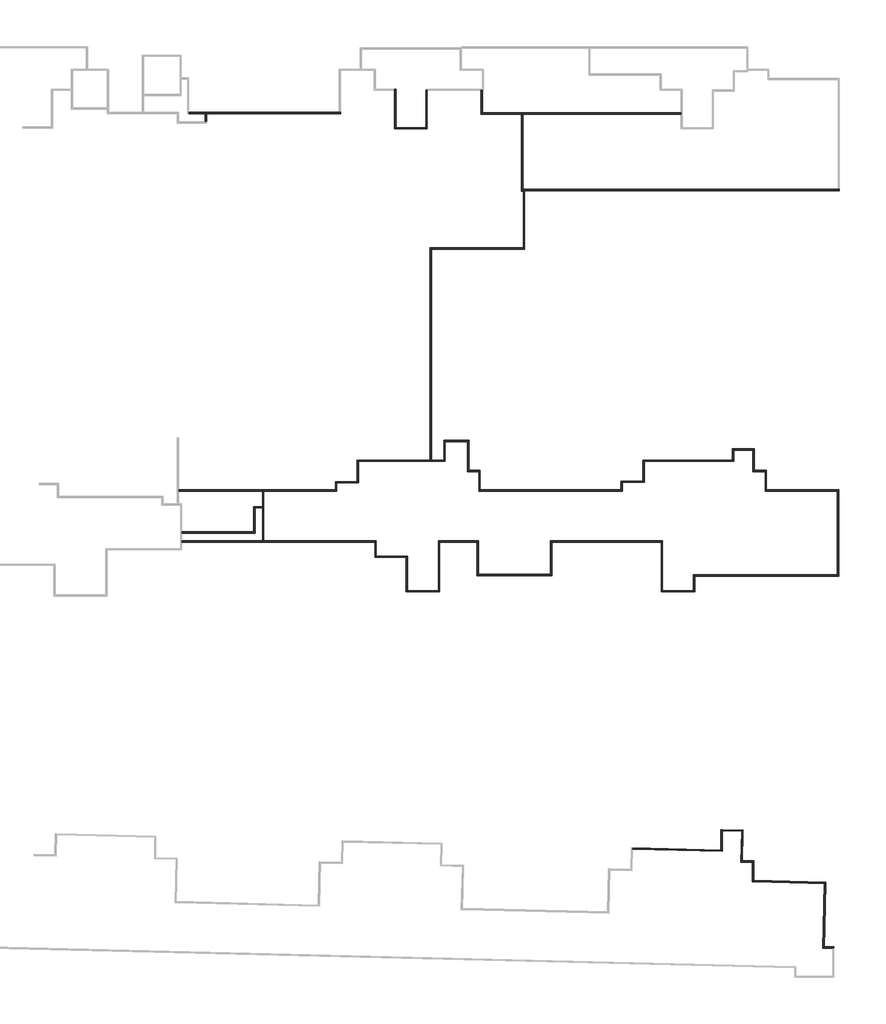
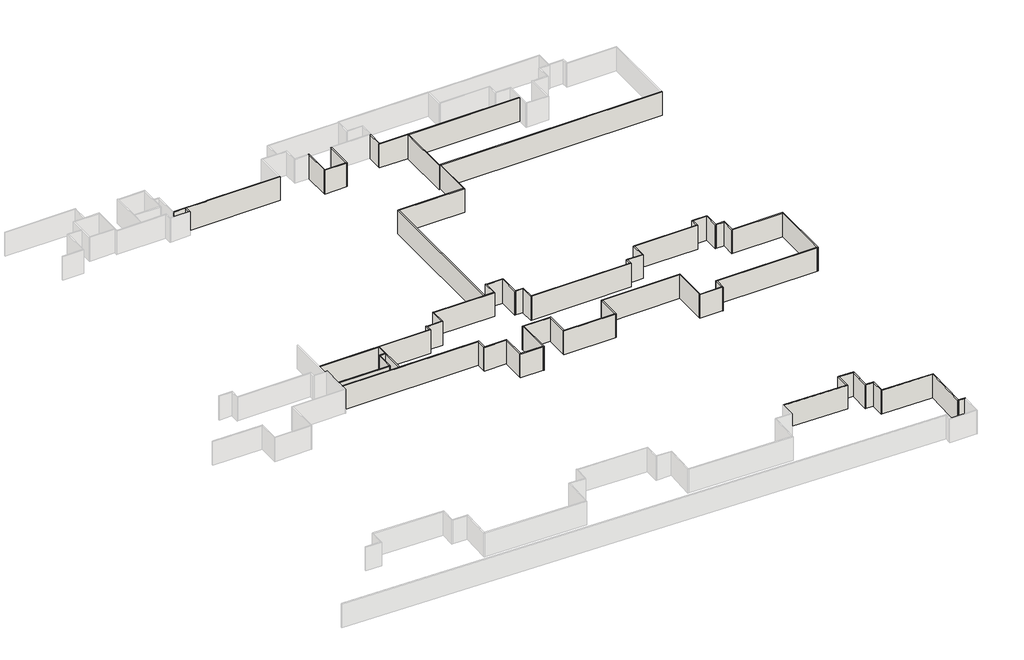
# One storey, part 7 of 8: 62 walls.
"""IFC4 building model written with IfcOpenShell, lengths in millimetres."""

from ifc_helpers import new_model, si_unit, origin, origin_with_axes, place, context, project, spatial, polyline, outline, extrude, faceted_brep, element, save

model = new_model("IFC4")

# Units and contexts
model_context = context("Model", 3, world=origin())
ifc_project = project(units=[si_unit("LENGTHUNIT", "METRE", prefix="MILLI")], contexts=[model_context])

# Site, building, storey
site = spatial("IfcSite", under=ifc_project)
building = spatial("IfcBuilding", under=site)
storey = spatial("IfcBuildingStorey", under=building, Name="户型图", Elevation=0.0)

# Walls
placement = place(None, origin())
element("IfcWall", 1, ObjectType="所有墙体", at=placement, inside=storey, context=model_context, shape_type="Brep", body=[
    faceted_brep([(295975.4891356, 26343.647248, 0.0), (304289.7878262, 26139.3963633, 0.0), (304289.7878262, 26139.3963633, 3300.0), (295975.4891356, 26343.647248, 3300.0), (295978.4361928, 26463.6110544, 0.0), (295978.4361928, 26463.6110544, 3300.0), (304169.7878262, 26262.3805141, 3300.0), (304289.7878262, 26259.4325678, 3300.0), (304289.7878262, 26259.4325678, 0.0), (304169.7878262, 26262.3805141, 0.0)], [[[0, 1, 2, 3]], [[4, 5, 6, 7, 8, 9]], [[1, 0, 4, 9, 8]], [[3, 2, 7, 6, 5]], [[0, 3, 5, 4]], [[2, 1, 8, 7]]]),
])
element("IfcWall", 2, ObjectType="所有墙体", at=placement, inside=storey, context=model_context, shape_type="Brep", body=[
    faceted_brep([(304289.7878262, 26259.4325678, 0.0), (304289.7878262, 28039.3963633, 0.0), (304289.7878262, 28159.4325678, 0.0), (304289.7878262, 28159.4325678, 3300.0), (304289.7878262, 28039.3963633, 3300.0), (304289.7878262, 26259.4325678, 3300.0), (304169.7878262, 26262.3805141, 0.0), (304169.7878262, 26262.3805141, 3300.0), (304169.7878262, 28162.3805141, 3300.0), (304169.7878262, 28162.3805141, 0.0)], [[[0, 1, 2, 3, 4, 5]], [[6, 7, 8, 9]], [[2, 1, 0, 6, 9]], [[5, 4, 3, 8, 7]], [[0, 5, 7, 6]], [[3, 2, 9, 8]]]),
])
element("IfcWall", 3, ObjectType="所有墙体", at=placement, inside=storey, context=model_context, shape_type="Brep", body=[
    faceted_brep([(304289.7878262, 28039.3963633, 0.0), (306114.4401038, 27994.5715553, 0.0), (306234.4039102, 27991.6244981, 0.0), (306234.4039102, 27991.6244981, 3300.0), (306114.4401038, 27994.5715553, 3300.0), (304289.7878262, 28039.3963633, 3300.0), (304289.7878262, 28159.4325678, 0.0), (304289.7878262, 28159.4325678, 3300.0), (306237.3509674, 28111.5883046, 3300.0), (306237.3509674, 28111.5883046, 0.0)], [[[0, 1, 2, 3, 4, 5]], [[6, 7, 8, 9]], [[2, 1, 0, 6, 9]], [[5, 4, 3, 8, 7]], [[0, 5, 7, 6]], [[3, 2, 9, 8]]]),
])
element("IfcWall", 4, ObjectType="所有墙体", at=placement, inside=storey, context=model_context, shape_type="Brep", body=[
    faceted_brep([(306114.4401038, 27994.5715553, 0.0), (306044.4174031, 25144.2061839, 0.0), (306044.4174031, 25144.2061839, 3300.0), (306114.4401038, 27994.5715553, 3300.0), (306234.4039102, 27991.6244981, 0.0), (306234.4039102, 27991.6244981, 3300.0), (306167.4015539, 25264.2061839, 3300.0), (306164.4536076, 25144.2061839, 3300.0), (306164.4536076, 25144.2061839, 0.0), (306167.4015539, 25264.2061839, 0.0)], [[[0, 1, 2, 3]], [[4, 5, 6, 7, 8, 9]], [[1, 0, 4, 9, 8]], [[3, 2, 7, 6, 5]], [[0, 3, 5, 4]], [[2, 1, 8, 7]]]),
])
element("IfcWall", 5, ObjectType="所有墙体", at=placement, inside=storey, context=model_context, shape_type="Brep", body=[
    faceted_brep([(306164.4536076, 25144.2061839, 0.0), (307105.9094785, 25144.2061839, 0.0), (307225.9094785, 25144.2061839, 0.0), (307225.9094785, 25144.2061839, 3300.0), (307105.9094785, 25144.2061839, 3300.0), (306164.4536076, 25144.2061839, 3300.0), (306167.4015539, 25264.2061839, 0.0), (306167.4015539, 25264.2061839, 3300.0), (307225.9094785, 25264.2061839, 3300.0), (307225.9094785, 25264.2061839, 0.0)], [[[0, 1, 2, 3, 4, 5]], [[6, 7, 8, 9]], [[2, 1, 0, 6, 9]], [[5, 4, 3, 8, 7]], [[0, 5, 7, 6]], [[3, 2, 9, 8]]]),
])
element("IfcWall", 6, ObjectType="所有墙体", at=placement, inside=storey, context=model_context, shape_type="Brep", body=[
    faceted_brep([(307105.9094785, 25144.2061839, 0.0), (307105.9094785, 23319.0782852, 0.0), (307105.9094785, 23319.0782852, 3300.0), (307105.9094785, 25144.2061839, 3300.0), (307225.9094785, 25144.2061839, 0.0), (307225.9094785, 25144.2061839, 3300.0), (307225.9094785, 23436.1665434, 3300.0), (307225.9094785, 23316.1303389, 3300.0), (307225.9094785, 23316.1303389, 0.0), (307225.9094785, 23436.1665434, 0.0)], [[[0, 1, 2, 3]], [[4, 5, 6, 7, 8, 9]], [[1, 0, 4, 9, 8]], [[3, 2, 7, 6, 5]], [[0, 3, 5, 4]], [[2, 1, 8, 7]]]),
])
element("IfcWall", 7, ObjectType="所有墙体", at=placement, inside=storey, context=model_context, shape_type="Brep", body=[
    faceted_brep([(307225.9094785, 23316.1303389, 0.0), (313802.4332392, 23154.5700142, 0.0), (313922.3970456, 23151.622957, 0.0), (313922.3970456, 23151.622957, 3300.0), (313802.4332392, 23154.5700142, 3300.0), (307225.9094785, 23316.1303389, 3300.0), (307225.9094785, 23436.1665434, 0.0), (307225.9094785, 23436.1665434, 3300.0), (313925.3441028, 23271.5867634, 3300.0), (313925.3441028, 23271.5867634, 0.0)], [[[0, 1, 2, 3, 4, 5]], [[6, 7, 8, 9]], [[2, 1, 0, 6, 9]], [[5, 4, 3, 8, 7]], [[0, 5, 7, 6]], [[3, 2, 9, 8]]]),
])
element("IfcWall", 8, ObjectType="所有墙体", at=placement, inside=storey, context=model_context, shape_type="Brep", body=[
    faceted_brep([(313802.4332392, 23154.5700142, 0.0), (313655.0436489, 17154.8844843, 0.0), (313655.0436489, 17154.8844843, 3300.0), (313802.4332392, 23154.5700142, 3300.0), (313922.3970456, 23151.622957, 0.0), (313922.3970456, 23151.622957, 3300.0), (313778.0277997, 17274.8844843, 3300.0), (313775.0798534, 17154.8844843, 3300.0), (313775.0798534, 17154.8844843, 0.0), (313778.0277997, 17274.8844843, 0.0)], [[[0, 1, 2, 3]], [[4, 5, 6, 7, 8, 9]], [[1, 0, 4, 9, 8]], [[3, 2, 7, 6, 5]], [[0, 3, 5, 4]], [[2, 1, 8, 7]]]),
])
element("IfcWall", 9, ObjectType="所有墙体", at=placement, inside=storey, context=model_context, shape_type="Brep", body=[
    faceted_brep([(313775.0798534, 17154.8844843, 0.0), (314556.5357243, 17154.8844843, 0.0), (314676.5357243, 17154.8844843, 0.0), (314676.5357243, 17154.8844843, 3300.0), (314556.5357243, 17154.8844843, 3300.0), (313775.0798534, 17154.8844843, 3300.0), (313778.0277997, 17274.8844843, 0.0), (313778.0277997, 17274.8844843, 3300.0), (314676.5357243, 17274.8844843, 3300.0), (314676.5357243, 17274.8844843, 0.0)], [[[0, 1, 2, 3, 4, 5]], [[6, 7, 8, 9]], [[2, 1, 0, 6, 9]], [[5, 4, 3, 8, 7]], [[0, 5, 7, 6]], [[3, 2, 9, 8]]]),
])
element("IfcWall", 10, ObjectType="所有墙体", at=placement, inside=storey, context=model_context, shape_type="SweptSolid", body=[
    extrude(outline(polyline([(256409.6849063, 94629.6848758), (256409.6849063, 93851.6486697), (256289.6849063, 93851.6486697), (256289.6849063, 94629.6848758), (256409.6849063, 94629.6848758)])), origin_with_axes(), (0.0, 0.0, 1.0), 3300.0),
])
element("IfcWall", 11, ObjectType="所有墙体", at=placement, inside=storey, context=model_context, shape_type="Brep", body=[
    faceted_brep([(254753.7757632, 94629.6848758, 0.0), (256289.6849063, 94629.6848758, 0.0), (256409.6849063, 94629.6848758, 0.0), (268831.7978195, 94629.6848758, 0.0), (268831.7978195, 94629.6848758, 2700.0), (268831.7978195, 94629.6848758, 3300.0), (268650.2438638, 94629.6848758, 3300.0), (259271.6890495, 94629.6848758, 3300.0), (258971.6890495, 94629.6848758, 3300.0), (256409.6849063, 94629.6848758, 3300.0), (256289.6849063, 94629.6848758, 3300.0), (254753.7757632, 94629.6848758, 3300.0), (254753.7757632, 94749.6848758, 0.0), (254753.7757632, 94749.6848758, 3300.0), (258971.6890495, 94749.6848758, 3300.0), (259271.6890495, 94749.6848758, 3300.0), (268711.7978195, 94749.6848758, 3300.0), (268831.7978195, 94749.6848758, 3300.0), (268831.7978195, 94749.6848758, 0.0), (268711.7978195, 94749.6848758, 0.0), (268831.7978195, 94694.4630172, 3300.0)], [[[0, 1, 2, 3, 4, 5, 6, 7, 8, 9, 10, 11]], [[12, 13, 14, 15, 16, 17, 18, 19]], [[3, 2, 1, 0, 12, 19, 18]], [[11, 10, 9, 8, 7, 6, 5, 20, 17, 16, 15, 14, 13]], [[5, 4, 3, 18, 17, 20]], [[0, 11, 13, 12]]]),
])
element("IfcWall", 12, ObjectType="所有墙体", at=placement, inside=storey, context=model_context, shape_type="Brep", body=[
    faceted_brep([(276761.765153, 96780.8975721, 0.0), (276761.765153, 93324.5302556, 0.0), (276761.765153, 93204.5302556, 0.0), (276761.765153, 93204.5302556, 3300.0), (276761.765153, 93324.5302556, 3300.0), (276761.765153, 96780.8975721, 3300.0), (276881.765153, 96780.8975721, 0.0), (276881.765153, 96780.8975721, 3300.0), (276881.765153, 93204.5302556, 3300.0), (276881.765153, 93204.5302556, 0.0)], [[[0, 1, 2, 3, 4, 5]], [[6, 7, 8, 9]], [[2, 1, 0, 6, 9]], [[5, 4, 3, 8, 7]], [[0, 5, 7, 6]], [[3, 2, 9, 8]]]),
])
element("IfcWall", 13, ObjectType="所有墙体", at=placement, inside=storey, context=model_context, shape_type="Brep", body=[
    faceted_brep([(276761.765153, 93324.5302556, 0.0), (273981.7651529, 93324.5302556, 0.0), (273861.7651529, 93324.5302556, 0.0), (273861.7651529, 93324.5302556, 3300.0), (273981.7651529, 93324.5302556, 3300.0), (276761.765153, 93324.5302556, 3300.0), (276761.765153, 93204.5302556, 0.0), (276761.765153, 93204.5302556, 3300.0), (273861.7651529, 93204.5302556, 3300.0), (273861.7651529, 93204.5302556, 0.0)], [[[0, 1, 2, 3, 4, 5]], [[6, 7, 8, 9]], [[2, 1, 0, 6, 9]], [[5, 4, 3, 8, 7]], [[0, 5, 7, 6]], [[3, 2, 9, 8]]]),
])
element("IfcWall", 14, ObjectType="所有墙体", at=placement, inside=storey, context=model_context, shape_type="Brep", body=[
    faceted_brep([(273981.7651529, 93324.5302556, 0.0), (273981.7651529, 96900.8975721, 0.0), (273981.7651529, 96900.8975721, 3300.0), (273981.7651529, 93324.5302556, 3300.0), (273861.7651529, 93324.5302556, 0.0), (273861.7651529, 93324.5302556, 3300.0), (273861.7651529, 96780.8975721, 3300.0), (273861.7651529, 96900.8975721, 3300.0), (273861.7651529, 96900.8975721, 0.0), (273861.7651529, 96780.8975721, 0.0)], [[[0, 1, 2, 3]], [[4, 5, 6, 7, 8, 9]], [[1, 0, 4, 9, 8]], [[3, 2, 7, 6, 5]], [[0, 3, 5, 4]], [[2, 1, 8, 7]]]),
])
element("IfcWall", 15, ObjectType="所有墙体", at=placement, inside=storey, context=model_context, shape_type="Brep", body=[
    faceted_brep([(253809.5875713, 59584.9975942, 0.0), (261588.0038327, 59584.9975942, 0.0), (261708.0038327, 59584.9975942, 0.0), (268485.4444886, 59584.9975942, 0.0), (268485.4444886, 59584.9975942, 3300.0), (261708.0038327, 59584.9975942, 3300.0), (261588.0038327, 59584.9975942, 3300.0), (253809.5875713, 59584.9975942, 3300.0), (253809.5875713, 59704.9975942, 0.0), (253809.5875713, 59704.9975942, 3300.0), (268365.4444886, 59704.9975942, 3300.0), (268485.4444886, 59704.9975942, 3300.0), (268485.4444886, 59704.9975942, 0.0), (268365.4444886, 59704.9975942, 0.0)], [[[0, 1, 2, 3, 4, 5, 6, 7]], [[8, 9, 10, 11, 12, 13]], [[3, 2, 1, 0, 8, 13, 12]], [[7, 6, 5, 4, 11, 10, 9]], [[4, 3, 12, 11]], [[0, 7, 9, 8]]]),
])
element("IfcWall", 16, ObjectType="所有墙体", at=placement, inside=storey, context=model_context, shape_type="Brep", body=[
    faceted_brep([(268485.4444886, 59704.9975942, 0.0), (268485.4444886, 60340.720191, 0.0), (268485.4444886, 60460.720191, 0.0), (268485.4444886, 60460.720191, 3300.0), (268485.4444886, 60340.720191, 3300.0), (268485.4444886, 59704.9975942, 3300.0), (268365.4444886, 59704.9975942, 0.0), (268365.4444886, 59704.9975942, 3300.0), (268365.4444886, 60460.720191, 3300.0), (268365.4444886, 60460.720191, 0.0)], [[[0, 1, 2, 3, 4, 5]], [[6, 7, 8, 9]], [[2, 1, 0, 6, 9]], [[5, 4, 3, 8, 7]], [[0, 5, 7, 6]], [[3, 2, 9, 8]]]),
])
element("IfcWall", 17, ObjectType="所有墙体", at=placement, inside=storey, context=model_context, shape_type="Brep", body=[
    faceted_brep([(268485.4444886, 60340.720191, 0.0), (270499.7227035, 60340.720191, 0.0), (270499.7227035, 60340.720191, 3300.0), (268485.4444886, 60340.720191, 3300.0), (268485.4444886, 60460.720191, 0.0), (268485.4444886, 60460.720191, 3300.0), (270379.7227035, 60460.720191, 3300.0), (270499.7227035, 60460.720191, 3300.0), (270499.7227035, 60460.720191, 0.0), (270379.7227035, 60460.720191, 0.0)], [[[0, 1, 2, 3]], [[4, 5, 6, 7, 8, 9]], [[1, 0, 4, 9, 8]], [[3, 2, 7, 6, 5]], [[0, 3, 5, 4]], [[2, 1, 8, 7]]]),
])
element("IfcWall", 18, ObjectType="所有墙体", at=placement, inside=storey, context=model_context, shape_type="Brep", body=[
    faceted_brep([(270499.7227035, 60460.720191, 0.0), (270499.7227035, 62334.5735496, 0.0), (270499.7227035, 62454.5735496, 0.0), (270499.7227035, 62454.5735496, 3300.0), (270499.7227035, 62334.5735496, 3300.0), (270499.7227035, 60460.720191, 3300.0), (270379.7227035, 60460.720191, 0.0), (270379.7227035, 60460.720191, 3300.0), (270379.7227035, 62423.9001534, 3300.0), (270379.7227035, 62454.5735496, 3300.0), (270379.7227035, 62454.5735496, 2700.0), (270379.7227035, 62454.5735496, 0.0), (270432.8505841, 62454.5735496, 3300.0)], [[[0, 1, 2, 3, 4, 5]], [[6, 7, 8, 9, 10, 11]], [[2, 1, 0, 6, 11]], [[5, 4, 3, 12, 9, 8, 7]], [[0, 5, 7, 6]], [[3, 2, 11, 10, 9, 12]]]),
])
element("IfcWall", 19, ObjectType="所有墙体", at=placement, inside=storey, context=model_context, shape_type="Brep", body=[
    faceted_brep([(270499.7227035, 62334.5735496, 0.0), (278560.2344713, 62334.5735496, 0.0), (278560.2344713, 62334.5735496, 3300.0), (270499.7227035, 62334.5735496, 3300.0), (270499.7227035, 62454.5735496, 0.0), (270499.7227035, 62454.5735496, 3300.0), (277178.9838503, 62454.5735496, 3300.0), (277298.9838503, 62454.5735496, 3300.0), (278440.2344713, 62454.5735496, 3300.0), (278560.2344713, 62454.5735496, 3300.0), (278560.2344713, 62454.5735496, 0.0), (278440.2344713, 62454.5735496, 0.0), (277298.9838503, 62454.5735496, 0.0), (277178.9838503, 62454.5735496, 0.0)], [[[0, 1, 2, 3]], [[4, 5, 6, 7, 8, 9, 10, 11, 12, 13]], [[1, 0, 4, 13, 12, 11, 10]], [[3, 2, 9, 8, 7, 6, 5]], [[0, 3, 5, 4]], [[2, 1, 10, 9]]]),
])
element("IfcWall", 20, ObjectType="所有墙体", at=placement, inside=storey, context=model_context, shape_type="Brep", body=[
    faceted_brep([(278560.2344713, 62454.5735496, 0.0), (278560.2344713, 64182.3314748, 0.0), (278560.2344713, 64302.3314748, 0.0), (278560.2344713, 64302.3314748, 3300.0), (278560.2344713, 64182.3314748, 3300.0), (278560.2344713, 62454.5735496, 3300.0), (278440.2344713, 62454.5735496, 0.0), (278440.2344713, 62454.5735496, 3300.0), (278440.2344713, 64302.3314748, 3300.0), (278440.2344713, 64302.3314748, 0.0)], [[[0, 1, 2, 3, 4, 5]], [[6, 7, 8, 9]], [[2, 1, 0, 6, 9]], [[5, 4, 3, 8, 7]], [[0, 5, 7, 6]], [[3, 2, 9, 8]]]),
])
element("IfcWall", 21, ObjectType="所有墙体", at=placement, inside=storey, context=model_context, shape_type="Brep", body=[
    faceted_brep([(278560.2344713, 64182.3314748, 0.0), (280640.2541721, 64182.3314748, 0.0), (280760.2541721, 64182.3314748, 0.0), (280760.2541721, 64182.3314748, 3300.0), (280640.2541721, 64182.3314748, 3300.0), (278560.2344713, 64182.3314748, 3300.0), (278560.2344713, 64302.3314748, 0.0), (278560.2344713, 64302.3314748, 3300.0), (280760.2541721, 64302.3314748, 3300.0), (280760.2541721, 64302.3314748, 0.0)], [[[0, 1, 2, 3, 4, 5]], [[6, 7, 8, 9]], [[2, 1, 0, 6, 9]], [[5, 4, 3, 8, 7]], [[0, 5, 7, 6]], [[3, 2, 9, 8]]]),
])
element("IfcWall", 22, ObjectType="所有墙体", at=placement, inside=storey, context=model_context, shape_type="Brep", body=[
    faceted_brep([(280640.2541721, 64182.3314748, 0.0), (280640.2541721, 61382.33135, 0.0), (280640.2541721, 61382.33135, 3300.0), (280640.2541721, 64182.3314748, 3300.0), (280760.2541721, 64182.3314748, 0.0), (280760.2541721, 64182.3314748, 3300.0), (280760.2541721, 61502.33135, 3300.0), (280760.2541721, 61382.33135, 3300.0), (280760.2541721, 61382.33135, 0.0), (280760.2541721, 61502.33135, 0.0)], [[[0, 1, 2, 3]], [[4, 5, 6, 7, 8, 9]], [[1, 0, 4, 9, 8]], [[3, 2, 7, 6, 5]], [[0, 3, 5, 4]], [[2, 1, 8, 7]]]),
])
element("IfcWall", 23, ObjectType="所有墙体", at=placement, inside=storey, context=model_context, shape_type="Brep", body=[
    faceted_brep([(280760.2541721, 61382.33135, 0.0), (281690.234471, 61382.33135, 0.0), (281810.234471, 61382.33135, 0.0), (281810.234471, 61382.33135, 3300.0), (281690.234471, 61382.33135, 3300.0), (280760.2541721, 61382.33135, 3300.0), (280760.2541721, 61502.33135, 0.0), (280760.2541721, 61502.33135, 3300.0), (281810.234471, 61502.33135, 3300.0), (281810.234471, 61502.33135, 0.0)], [[[0, 1, 2, 3, 4, 5]], [[6, 7, 8, 9]], [[2, 1, 0, 6, 9]], [[5, 4, 3, 8, 7]], [[0, 5, 7, 6]], [[3, 2, 9, 8]]]),
])
element("IfcWall", 24, ObjectType="所有墙体", at=placement, inside=storey, context=model_context, shape_type="Brep", body=[
    faceted_brep([(281690.234471, 61382.33135, 0.0), (281690.234471, 59584.9975942, 0.0), (281690.234471, 59584.9975942, 3300.0), (281690.234471, 61382.33135, 3300.0), (281810.234471, 61382.33135, 0.0), (281810.234471, 61382.33135, 3300.0), (281810.234471, 59704.9975942, 3300.0), (281810.234471, 59584.9975942, 3300.0), (281810.234471, 59584.9975942, 0.0), (281810.234471, 59704.9975942, 0.0)], [[[0, 1, 2, 3]], [[4, 5, 6, 7, 8, 9]], [[1, 0, 4, 9, 8]], [[3, 2, 7, 6, 5]], [[0, 3, 5, 4]], [[2, 1, 8, 7]]]),
])
element("IfcWall", 25, ObjectType="所有墙体", at=placement, inside=storey, context=model_context, shape_type="Brep", body=[
    faceted_brep([(281810.234471, 59584.9975942, 0.0), (295010.2344624, 59584.9975942, 0.0), (295010.2344624, 59584.9975942, 3300.0), (281810.234471, 59584.9975942, 3300.0), (281810.234471, 59704.9975942, 0.0), (281810.234471, 59704.9975942, 3300.0), (294890.2344624, 59704.9975942, 3300.0), (295010.2344624, 59704.9975942, 3300.0), (295010.2344624, 59704.9975942, 0.0), (294890.2344624, 59704.9975942, 0.0)], [[[0, 1, 2, 3]], [[4, 5, 6, 7, 8, 9]], [[1, 0, 4, 9, 8]], [[3, 2, 7, 6, 5]], [[0, 3, 5, 4]], [[2, 1, 8, 7]]]),
])
element("IfcWall", 26, ObjectType="所有墙体", at=placement, inside=storey, context=model_context, shape_type="Brep", body=[
    faceted_brep([(295010.2344624, 59704.9975942, 0.0), (295010.2344624, 60382.7613824, 0.0), (295010.2344624, 60502.7613824, 0.0), (295010.2344624, 60502.7613824, 3300.0), (295010.2344624, 60382.7613824, 3300.0), (295010.2344624, 59704.9975942, 3300.0), (294890.2344624, 59704.9975942, 0.0), (294890.2344624, 59704.9975942, 3300.0), (294890.2344624, 60502.7613824, 3300.0), (294890.2344624, 60502.7613824, 0.0)], [[[0, 1, 2, 3, 4, 5]], [[6, 7, 8, 9]], [[2, 1, 0, 6, 9]], [[5, 4, 3, 8, 7]], [[0, 5, 7, 6]], [[3, 2, 9, 8]]]),
])
element("IfcWall", 27, ObjectType="所有墙体", at=placement, inside=storey, context=model_context, shape_type="Brep", body=[
    faceted_brep([(295010.2344624, 60382.7613824, 0.0), (297060.2344614, 60382.7613824, 0.0), (297060.2344614, 60382.7613824, 3300.0), (295010.2344624, 60382.7613824, 3300.0), (295010.2344624, 60502.7613824, 0.0), (295010.2344624, 60502.7613824, 3300.0), (296940.2344614, 60502.7613824, 3300.0), (297060.2344614, 60502.7613824, 3300.0), (297060.2344614, 60502.7613824, 0.0), (296940.2344614, 60502.7613824, 0.0)], [[[0, 1, 2, 3]], [[4, 5, 6, 7, 8, 9]], [[1, 0, 4, 9, 8]], [[3, 2, 7, 6, 5]], [[0, 3, 5, 4]], [[2, 1, 8, 7]]]),
])
element("IfcWall", 28, ObjectType="所有墙体", at=placement, inside=storey, context=model_context, shape_type="Brep", body=[
    faceted_brep([(297060.2344614, 60502.7613824, 0.0), (297060.2344614, 62334.5735496, 0.0), (297060.2344614, 62454.5735496, 0.0), (297060.2344614, 62454.5735496, 3300.0), (297060.2344614, 62334.5735496, 3300.0), (297060.2344614, 60502.7613824, 3300.0), (296940.2344614, 60502.7613824, 0.0), (296940.2344614, 60502.7613824, 3300.0), (296940.2344614, 62454.5735496, 3300.0), (296940.2344614, 62454.5735496, 0.0)], [[[0, 1, 2, 3, 4, 5]], [[6, 7, 8, 9]], [[2, 1, 0, 6, 9]], [[5, 4, 3, 8, 7]], [[0, 5, 7, 6]], [[3, 2, 9, 8]]]),
])
element("IfcWall", 29, ObjectType="所有墙体", at=placement, inside=storey, context=model_context, shape_type="Brep", body=[
    faceted_brep([(297060.2344614, 62334.5735496, 0.0), (305360.2304568, 62334.5735496, 0.0), (305360.2304568, 62334.5735496, 3300.0), (297060.2344614, 62334.5735496, 3300.0), (297060.2344614, 62454.5735496, 0.0), (297060.2344614, 62454.5735496, 3300.0), (305240.2304568, 62454.5735496, 3300.0), (305360.2304568, 62454.5735496, 3300.0), (305360.2304568, 62454.5735496, 0.0), (305240.2304568, 62454.5735496, 0.0)], [[[0, 1, 2, 3]], [[4, 5, 6, 7, 8, 9]], [[1, 0, 4, 9, 8]], [[3, 2, 7, 6, 5]], [[0, 3, 5, 4]], [[2, 1, 8, 7]]]),
])
element("IfcWall", 30, ObjectType="所有墙体", at=placement, inside=storey, context=model_context, shape_type="Brep", body=[
    faceted_brep([(305360.2304568, 62454.5735496, 0.0), (305360.2304568, 63382.3074511, 0.0), (305360.2304568, 63502.3074511, 0.0), (305360.2304568, 63502.3074511, 3300.0), (305360.2304568, 63382.3074511, 3300.0), (305360.2304568, 62454.5735496, 3300.0), (305240.2304568, 62454.5735496, 0.0), (305240.2304568, 62454.5735496, 3300.0), (305240.2304568, 63502.3074511, 3300.0), (305240.2304568, 63502.3074511, 0.0)], [[[0, 1, 2, 3, 4, 5]], [[6, 7, 8, 9]], [[2, 1, 0, 6, 9]], [[5, 4, 3, 8, 7]], [[0, 5, 7, 6]], [[3, 2, 9, 8]]]),
])
element("IfcWall", 31, ObjectType="所有墙体", at=placement, inside=storey, context=model_context, shape_type="Brep", body=[
    faceted_brep([(305360.2304568, 63382.3074511, 0.0), (307140.2304762, 63382.3074511, 0.0), (307260.2304762, 63382.3074511, 0.0), (307260.2304762, 63382.3074511, 3300.0), (307140.2304762, 63382.3074511, 3300.0), (305360.2304568, 63382.3074511, 3300.0), (305360.2304568, 63502.3074511, 0.0), (305360.2304568, 63502.3074511, 3300.0), (307260.2304762, 63502.3074511, 3300.0), (307260.2304762, 63502.3074511, 0.0)], [[[0, 1, 2, 3, 4, 5]], [[6, 7, 8, 9]], [[2, 1, 0, 6, 9]], [[5, 4, 3, 8, 7]], [[0, 5, 7, 6]], [[3, 2, 9, 8]]]),
])
element("IfcWall", 32, ObjectType="所有墙体", at=placement, inside=storey, context=model_context, shape_type="Brep", body=[
    faceted_brep([(307140.2304762, 63382.3074511, 0.0), (307140.2304762, 61382.3313458, 0.0), (307140.2304762, 61382.3313458, 3300.0), (307140.2304762, 63382.3074511, 3300.0), (307260.2304762, 63382.3074511, 0.0), (307260.2304762, 63382.3074511, 3300.0), (307260.2304762, 61502.3313458, 3300.0), (307260.2304762, 61382.3313458, 3300.0), (307260.2304762, 61382.3313458, 0.0), (307260.2304762, 61502.3313458, 0.0)], [[[0, 1, 2, 3]], [[4, 5, 6, 7, 8, 9]], [[1, 0, 4, 9, 8]], [[3, 2, 7, 6, 5]], [[0, 3, 5, 4]], [[2, 1, 8, 7]]]),
])
element("IfcWall", 33, ObjectType="所有墙体", at=placement, inside=storey, context=model_context, shape_type="Brep", body=[
    faceted_brep([(307260.2304762, 61382.3313458, 0.0), (308290.2344624, 61382.3313458, 0.0), (308410.2344624, 61382.3313458, 0.0), (308410.2344624, 61382.3313458, 3300.0), (308290.2344624, 61382.3313458, 3300.0), (307260.2304762, 61382.3313458, 3300.0), (307260.2304762, 61502.3313458, 0.0), (307260.2304762, 61502.3313458, 3300.0), (308410.2344624, 61502.3313458, 3300.0), (308410.2344624, 61502.3313458, 0.0)], [[[0, 1, 2, 3, 4, 5]], [[6, 7, 8, 9]], [[2, 1, 0, 6, 9]], [[5, 4, 3, 8, 7]], [[0, 5, 7, 6]], [[3, 2, 9, 8]]]),
])
element("IfcWall", 34, ObjectType="所有墙体", at=placement, inside=storey, context=model_context, shape_type="Brep", body=[
    faceted_brep([(308290.2344624, 61382.3313458, 0.0), (308290.2344624, 59584.9975942, 0.0), (308290.2344624, 59584.9975942, 3300.0), (308290.2344624, 61382.3313458, 3300.0), (308410.2344624, 61382.3313458, 0.0), (308410.2344624, 61382.3313458, 3300.0), (308410.2344624, 59704.9975942, 3300.0), (308410.2344624, 59584.9975942, 3300.0), (308410.2344624, 59584.9975942, 0.0), (308410.2344624, 59704.9975942, 0.0)], [[[0, 1, 2, 3]], [[4, 5, 6, 7, 8, 9]], [[1, 0, 4, 9, 8]], [[3, 2, 7, 6, 5]], [[0, 3, 5, 4]], [[2, 1, 8, 7]]]),
])
element("IfcWall", 35, ObjectType="所有墙体", at=placement, inside=storey, context=model_context, shape_type="Brep", body=[
    faceted_brep([(308410.2344624, 59584.9975942, 0.0), (314990.2344624, 59584.9975942, 0.0), (315110.2344624, 59584.9975942, 0.0), (315110.2344624, 59584.9975942, 3300.0), (314990.2344624, 59584.9975942, 3300.0), (308410.2344624, 59584.9975942, 3300.0), (308410.2344624, 59704.9975942, 0.0), (308410.2344624, 59704.9975942, 3300.0), (315110.2344624, 59704.9975942, 3300.0), (315110.2344624, 59704.9975942, 0.0)], [[[0, 1, 2, 3, 4, 5]], [[6, 7, 8, 9]], [[2, 1, 0, 6, 9]], [[5, 4, 3, 8, 7]], [[0, 5, 7, 6]], [[3, 2, 9, 8]]]),
])
element("IfcWall", 36, ObjectType="所有墙体", at=placement, inside=storey, context=model_context, shape_type="Brep", body=[
    faceted_brep([(314990.2344624, 59584.9975942, 0.0), (314990.2344624, 51802.3314613, 0.0), (314990.2344624, 51682.3314613, 0.0), (314990.2344624, 51682.3314613, 3300.0), (314990.2344624, 51802.3314613, 3300.0), (314990.2344624, 59584.9975942, 3300.0), (315110.2344624, 59584.9975942, 0.0), (315110.2344624, 59584.9975942, 3300.0), (315110.2344624, 51682.3314613, 3300.0), (315110.2344624, 51682.3314613, 0.0)], [[[0, 1, 2, 3, 4, 5]], [[6, 7, 8, 9]], [[2, 1, 0, 6, 9]], [[5, 4, 3, 8, 7]], [[0, 5, 7, 6]], [[3, 2, 9, 8]]]),
])
element("IfcWall", 37, ObjectType="所有墙体", at=placement, inside=storey, context=model_context, shape_type="Brep", body=[
    faceted_brep([(314990.2344624, 51802.3314613, 0.0), (301640.3717048, 51802.3314613, 0.0), (301640.3717048, 51802.3314613, 3300.0), (314990.2344624, 51802.3314613, 3300.0), (314990.2344624, 51682.3314613, 0.0), (314990.2344624, 51682.3314613, 3300.0), (301760.3717048, 51682.3314613, 3300.0), (301640.3717048, 51682.3314613, 3300.0), (301640.3717048, 51682.3314613, 0.0), (301760.3717048, 51682.3314613, 0.0)], [[[0, 1, 2, 3]], [[4, 5, 6, 7, 8, 9]], [[1, 0, 4, 9, 8]], [[3, 2, 7, 6, 5]], [[0, 3, 5, 4]], [[2, 1, 8, 7]]]),
])
element("IfcWall", 38, ObjectType="所有墙体", at=placement, inside=storey, context=model_context, shape_type="Brep", body=[
    faceted_brep([(301640.3717048, 51682.3314613, 0.0), (301640.3717048, 50352.3314615, 0.0), (301640.3717048, 50232.3314615, 0.0), (301640.3717048, 50232.3314615, 3300.0), (301640.3717048, 50352.3314615, 3300.0), (301640.3717048, 51682.3314613, 3300.0), (301760.3717048, 51682.3314613, 0.0), (301760.3717048, 51682.3314613, 3300.0), (301760.3717048, 50232.3314615, 3300.0), (301760.3717048, 50232.3314615, 0.0)], [[[0, 1, 2, 3, 4, 5]], [[6, 7, 8, 9]], [[2, 1, 0, 6, 9]], [[5, 4, 3, 8, 7]], [[0, 5, 7, 6]], [[3, 2, 9, 8]]]),
])
element("IfcWall", 39, ObjectType="所有墙体", at=placement, inside=storey, context=model_context, shape_type="Brep", body=[
    faceted_brep([(301640.3717048, 50352.3314615, 0.0), (298760.3716961, 50352.3314615, 0.0), (298640.3716961, 50352.3314615, 0.0), (298640.3716961, 50352.3314615, 3300.0), (298760.3716961, 50352.3314615, 3300.0), (301640.3717048, 50352.3314615, 3300.0), (301640.3717048, 50232.3314615, 0.0), (301640.3717048, 50232.3314615, 3300.0), (298640.3716961, 50232.3314615, 3300.0), (298640.3716961, 50232.3314615, 0.0)], [[[0, 1, 2, 3, 4, 5]], [[6, 7, 8, 9]], [[2, 1, 0, 6, 9]], [[5, 4, 3, 8, 7]], [[0, 5, 7, 6]], [[3, 2, 9, 8]]]),
])
element("IfcWall", 40, ObjectType="所有墙体", at=placement, inside=storey, context=model_context, shape_type="Brep", body=[
    faceted_brep([(298760.3716961, 50352.3314615, 0.0), (298760.3716961, 54952.3246977, 0.0), (298760.3716961, 54952.3246977, 3300.0), (298760.3716961, 50352.3314615, 3300.0), (298640.3716961, 50352.3314615, 0.0), (298640.3716961, 50352.3314615, 3300.0), (298640.3716961, 54832.3246977, 3300.0), (298640.3716961, 54952.3246977, 3300.0), (298640.3716961, 54952.3246977, 0.0), (298640.3716961, 54832.3246977, 0.0)], [[[0, 1, 2, 3]], [[4, 5, 6, 7, 8, 9]], [[1, 0, 4, 9, 8]], [[3, 2, 7, 6, 5]], [[0, 3, 5, 4]], [[2, 1, 8, 7]]]),
])
element("IfcWall", 41, ObjectType="所有墙体", at=placement, inside=storey, context=model_context, shape_type="Brep", body=[
    faceted_brep([(298640.3716961, 54952.3246977, 0.0), (288340.2344711, 54952.3246977, 0.0), (288340.2344711, 54952.3246977, 3300.0), (298640.3716961, 54952.3246977, 3300.0), (298640.3716961, 54832.3246977, 0.0), (298640.3716961, 54832.3246977, 3300.0), (288460.2344711, 54832.3246977, 3300.0), (288340.2344711, 54832.3246977, 3300.0), (288340.2344711, 54832.3246977, 0.0), (288460.2344711, 54832.3246977, 0.0)], [[[0, 1, 2, 3]], [[4, 5, 6, 7, 8, 9]], [[1, 0, 4, 9, 8]], [[3, 2, 7, 6, 5]], [[0, 3, 5, 4]], [[2, 1, 8, 7]]]),
])
element("IfcWall", 42, ObjectType="所有墙体", at=placement, inside=storey, context=model_context, shape_type="Brep", body=[
    faceted_brep([(288340.2344711, 54832.3246977, 0.0), (288340.2344711, 51852.3246977, 0.0), (288340.2344711, 51732.3246977, 0.0), (288340.2344711, 51732.3246977, 3300.0), (288340.2344711, 51852.3246977, 3300.0), (288340.2344711, 54832.3246977, 3300.0), (288460.2344711, 54832.3246977, 0.0), (288460.2344711, 54832.3246977, 3300.0), (288460.2344711, 51852.3246977, 3300.0), (288460.2344711, 51732.3246977, 3300.0), (288460.2344711, 51732.3246977, 2700.0), (288460.2344711, 51732.3246977, 0.0)], [[[0, 1, 2, 3, 4, 5]], [[6, 7, 8, 9, 10, 11]], [[2, 1, 0, 6, 11]], [[5, 4, 3, 9, 8, 7]], [[0, 5, 7, 6]], [[3, 2, 11, 10, 9]]]),
])
element("IfcWall", 43, ObjectType="所有墙体", at=placement, inside=storey, context=model_context, shape_type="Brep", body=[
    faceted_brep([(288340.2344711, 51852.3246977, 0.0), (281660.2344711, 51852.3246977, 0.0), (281540.2344711, 51852.3246977, 0.0), (281540.2344711, 51852.3246977, 3300.0), (281660.2344711, 51852.3246977, 3300.0), (288340.2344711, 51852.3246977, 3300.0), (288340.2344711, 51732.3246977, 0.0), (288340.2344711, 51732.3246977, 3300.0), (281663.9582145, 51732.3246977, 3300.0), (281540.2344711, 51732.3246977, 3300.0), (281540.2344711, 51732.3246977, 2700.0), (281540.2344711, 51732.3246977, 0.0), (281540.2344711, 51842.0227808, 3300.0)], [[[0, 1, 2, 3, 4, 5]], [[6, 7, 8, 9, 10, 11]], [[2, 1, 0, 6, 11]], [[5, 4, 3, 12, 9, 8, 7]], [[0, 5, 7, 6]], [[3, 2, 11, 10, 9, 12]]]),
])
element("IfcWall", 44, ObjectType="所有墙体", at=placement, inside=storey, context=model_context, shape_type="Brep", body=[
    faceted_brep([(281660.2344711, 51852.3246977, 0.0), (281660.2344711, 54952.3246977, 0.0), (281660.2344711, 54952.3246977, 3300.0), (281660.2344711, 51852.3246977, 3300.0), (281540.2344711, 51852.3246977, 0.0), (281540.2344711, 51852.3246977, 3300.0), (281540.2344711, 54832.3246977, 3300.0), (281540.2344711, 54952.3246977, 3300.0), (281540.2344711, 54952.3246977, 0.0), (281540.2344711, 54832.3246977, 0.0)], [[[0, 1, 2, 3]], [[4, 5, 6, 7, 8, 9]], [[1, 0, 4, 9, 8]], [[3, 2, 7, 6, 5]], [[0, 3, 5, 4]], [[2, 1, 8, 7]]]),
])
element("IfcWall", 45, ObjectType="所有墙体", at=placement, inside=storey, context=model_context, shape_type="Brep", body=[
    faceted_brep([(281540.2344711, 54952.3246977, 0.0), (277940.3720183, 54952.3246977, 0.0), (277940.3720183, 54952.3246977, 3300.0), (281540.2344711, 54952.3246977, 3300.0), (281540.2344711, 54832.3246977, 0.0), (281540.2344711, 54832.3246977, 3300.0), (278060.3720183, 54832.3246977, 3300.0), (277940.3720183, 54832.3246977, 3300.0), (277940.3720183, 54832.3246977, 0.0), (278060.3720183, 54832.3246977, 0.0)], [[[0, 1, 2, 3]], [[4, 5, 6, 7, 8, 9]], [[1, 0, 4, 9, 8]], [[3, 2, 7, 6, 5]], [[0, 3, 5, 4]], [[2, 1, 8, 7]]]),
])
element("IfcWall", 46, ObjectType="所有墙体", at=placement, inside=storey, context=model_context, shape_type="Brep", body=[
    faceted_brep([(277940.3720183, 54832.3246977, 0.0), (277940.3720183, 50352.3314615, 0.0), (277940.3720183, 50232.3314615, 0.0), (277940.3720183, 50232.3314615, 3300.0), (277940.3720183, 50352.3314615, 3300.0), (277940.3720183, 54832.3246977, 3300.0), (278060.3720183, 54832.3246977, 0.0), (278060.3720183, 54832.3246977, 3300.0), (278060.3720183, 50232.3314615, 3300.0), (278060.3720183, 50232.3314615, 0.0)], [[[0, 1, 2, 3, 4, 5]], [[6, 7, 8, 9]], [[2, 1, 0, 6, 9]], [[5, 4, 3, 8, 7]], [[0, 5, 7, 6]], [[3, 2, 9, 8]]]),
])
element("IfcWall", 47, ObjectType="所有墙体", at=placement, inside=storey, context=model_context, shape_type="Brep", body=[
    faceted_brep([(277940.3720183, 50352.3314615, 0.0), (275060.3720183, 50352.3314615, 0.0), (274940.3720183, 50352.3314615, 0.0), (274940.3720183, 50352.3314615, 3300.0), (275060.3720183, 50352.3314615, 3300.0), (277940.3720183, 50352.3314615, 3300.0), (277940.3720183, 50232.3314615, 0.0), (277940.3720183, 50232.3314615, 3300.0), (275149.8189959, 50232.3314615, 3300.0), (274940.3720183, 50232.3314615, 3300.0), (274940.3720183, 50232.3314615, 2700.0), (274940.3720183, 50232.3314615, 0.0), (274940.3720183, 50321.8046245, 3300.0)], [[[0, 1, 2, 3, 4, 5]], [[6, 7, 8, 9, 10, 11]], [[2, 1, 0, 6, 11]], [[5, 4, 3, 12, 9, 8, 7]], [[0, 5, 7, 6]], [[3, 2, 11, 10, 9, 12]]]),
])
element("IfcWall", 48, ObjectType="所有墙体", at=placement, inside=storey, context=model_context, shape_type="Brep", body=[
    faceted_brep([(275060.3720183, 50352.3314615, 0.0), (275060.3720183, 53552.324698, 0.0), (275060.3720183, 53552.324698, 3300.0), (275060.3720183, 50352.3314615, 3300.0), (274940.3720183, 50352.3314615, 0.0), (274940.3720183, 50352.3314615, 3300.0), (274940.3720183, 53432.324698, 3300.0), (274940.3720183, 53552.324698, 3300.0), (274940.3720183, 53552.324698, 0.0), (274940.3720183, 53432.324698, 0.0)], [[[0, 1, 2, 3]], [[4, 5, 6, 7, 8, 9]], [[1, 0, 4, 9, 8]], [[3, 2, 7, 6, 5]], [[0, 3, 5, 4]], [[2, 1, 8, 7]]]),
])
element("IfcWall", 49, ObjectType="所有墙体", at=placement, inside=storey, context=model_context, shape_type="Brep", body=[
    faceted_brep([(274940.3720183, 53552.324698, 0.0), (272160.3717048, 53552.324698, 0.0), (272040.3717048, 53552.324698, 0.0), (272040.3717048, 53552.324698, 3300.0), (272160.3717048, 53552.324698, 3300.0), (274940.3720183, 53552.324698, 3300.0), (274940.3720183, 53432.324698, 0.0), (274940.3720183, 53432.324698, 3300.0), (272040.3717048, 53432.324698, 3300.0), (272040.3717048, 53432.324698, 0.0)], [[[0, 1, 2, 3, 4, 5]], [[6, 7, 8, 9]], [[2, 1, 0, 6, 9]], [[5, 4, 3, 8, 7]], [[0, 5, 7, 6]], [[3, 2, 9, 8]]]),
])
element("IfcWall", 50, ObjectType="所有墙体", at=placement, inside=storey, context=model_context, shape_type="Brep", body=[
    faceted_brep([(272160.3717048, 53552.324698, 0.0), (272160.3717048, 54952.3246977, 0.0), (272160.3717048, 54952.3246977, 3300.0), (272160.3717048, 53552.324698, 3300.0), (272040.3717048, 53552.324698, 0.0), (272040.3717048, 53552.324698, 3300.0), (272040.3717048, 54832.3246977, 3300.0), (272040.3717048, 54952.3246977, 3300.0), (272040.3717048, 54952.3246977, 0.0), (272040.3717048, 54832.3246977, 0.0)], [[[0, 1, 2, 3]], [[4, 5, 6, 7, 8, 9]], [[1, 0, 4, 9, 8]], [[3, 2, 7, 6, 5]], [[0, 3, 5, 4]], [[2, 1, 8, 7]]]),
])
element("IfcWall", 51, ObjectType="所有墙体", at=placement, inside=storey, context=model_context, shape_type="Brep", body=[
    faceted_brep([(272040.3717048, 54952.3246977, 0.0), (261708.0038327, 54952.3246977, 0.0), (261588.0038327, 54952.3246977, 0.0), (254109.7167317, 54952.3246977, 0.0), (254109.7167317, 54952.3246977, 3300.0), (261588.0038327, 54952.3246977, 3300.0), (261708.0038327, 54952.3246977, 3300.0), (272040.3717048, 54952.3246977, 3300.0), (272040.3717048, 54832.3246977, 0.0), (272040.3717048, 54832.3246977, 3300.0), (254109.7167317, 54832.3246977, 3300.0), (254109.7167317, 54832.3246977, 0.0)], [[[0, 1, 2, 3, 4, 5, 6, 7]], [[8, 9, 10, 11]], [[3, 2, 1, 0, 8, 11]], [[7, 6, 5, 4, 10, 9]], [[0, 7, 9, 8]], [[4, 3, 11, 10]]]),
])
element("IfcWall", 52, ObjectType="所有墙体", at=placement, inside=storey, context=model_context, shape_type="Brep", body=[
    faceted_brep([(261708.0038327, 54952.3246977, 0.0), (261708.0038327, 59584.9975942, 0.0), (261708.0038327, 59584.9975942, 3300.0), (261708.0038327, 54952.3246977, 3300.0), (261588.0038327, 54952.3246977, 0.0), (261588.0038327, 54952.3246977, 3300.0), (261588.0038327, 58032.3226853, 3300.0), (261588.0038327, 58152.3226853, 3300.0), (261588.0038327, 59584.9975942, 3300.0), (261588.0038327, 59584.9975942, 0.0), (261588.0038327, 58152.3226853, 0.0), (261588.0038327, 58032.3226853, 0.0)], [[[0, 1, 2, 3]], [[4, 5, 6, 7, 8, 9, 10, 11]], [[1, 0, 4, 11, 10, 9]], [[3, 2, 8, 7, 6, 5]], [[0, 3, 5, 4]], [[2, 1, 9, 8]]]),
])
element("IfcWall", 53, ObjectType="所有墙体", at=placement, inside=storey, context=model_context, shape_type="Brep", body=[
    faceted_brep([(261588.0038327, 58152.3226853, 0.0), (260790.2003011, 58152.3226853, 0.0), (260790.2003011, 58152.3226853, 3300.0), (261588.0038327, 58152.3226853, 3300.0), (261588.0038327, 58032.3226853, 0.0), (261588.0038327, 58032.3226853, 3300.0), (260910.2003011, 58032.3226853, 3300.0), (260790.2003011, 58032.3226853, 3300.0), (260790.2003011, 58032.3226853, 0.0), (260910.2003011, 58032.3226853, 0.0)], [[[0, 1, 2, 3]], [[4, 5, 6, 7, 8, 9]], [[1, 0, 4, 9, 8]], [[3, 2, 7, 6, 5]], [[0, 3, 5, 4]], [[2, 1, 8, 7]]]),
])
element("IfcWall", 54, ObjectType="所有墙体", at=placement, inside=storey, context=model_context, shape_type="Brep", body=[
    faceted_brep([(260790.2003011, 58032.3226853, 0.0), (260790.2003011, 55802.3681078, 0.0), (260790.2003011, 55682.3681078, 0.0), (260790.2003011, 55682.3681078, 3300.0), (260790.2003011, 55802.3681078, 3300.0), (260790.2003011, 58032.3226853, 3300.0), (260910.2003011, 58032.3226853, 0.0), (260910.2003011, 58032.3226853, 3300.0), (260910.2003011, 55682.3681078, 3300.0), (260910.2003011, 55682.3681078, 0.0)], [[[0, 1, 2, 3, 4, 5]], [[6, 7, 8, 9]], [[2, 1, 0, 6, 9]], [[5, 4, 3, 8, 7]], [[0, 5, 7, 6]], [[3, 2, 9, 8]]]),
])
element("IfcWall", 55, ObjectType="所有墙体", at=placement, inside=storey, context=model_context, shape_type="SweptSolid", body=[
    extrude(outline(polyline([(254109.7167317, 55802.3681078), (260790.2003011, 55802.3681078), (260790.2003011, 55682.3681078), (254109.7167317, 55682.3681078), (254109.7167317, 55802.3681078)])), origin_with_axes(), (0.0, 0.0, 1.0), 3300.0),
])
element("IfcWall", 56, ObjectType="所有墙体", at=placement, inside=storey, context=model_context, shape_type="Brep", body=[
    faceted_brep([(277298.9838503, 62454.5735496, 0.0), (277298.9838503, 82034.5735496, 0.0), (277298.9838503, 82154.5735496, 0.0), (277298.9838503, 82154.5735496, 3300.0), (277298.9838503, 82034.5735496, 3300.0), (277298.9838503, 62454.5735496, 3300.0), (277178.9838503, 62454.5735496, 0.0), (277178.9838503, 62454.5735496, 3300.0), (277178.9838503, 82154.5735496, 3300.0), (277178.9838503, 82154.5735496, 0.0)], [[[0, 1, 2, 3, 4, 5]], [[6, 7, 8, 9]], [[2, 1, 0, 6, 9]], [[5, 4, 3, 8, 7]], [[0, 5, 7, 6]], [[3, 2, 9, 8]]]),
])
element("IfcWall", 57, ObjectType="所有墙体", at=placement, inside=storey, context=model_context, shape_type="Brep", body=[
    faceted_brep([(277298.9838503, 82034.5735496, 0.0), (285938.3344634, 82034.5735496, 0.0), (285938.3344634, 82034.5735496, 3300.0), (277298.9838503, 82034.5735496, 3300.0), (277298.9838503, 82154.5735496, 0.0), (277298.9838503, 82154.5735496, 3300.0), (285818.3344634, 82154.5735496, 3300.0), (285938.3344634, 82154.5735496, 3300.0), (285938.3344634, 82154.5735496, 0.0), (285818.3344634, 82154.5735496, 0.0)], [[[0, 1, 2, 3]], [[4, 5, 6, 7, 8, 9]], [[1, 0, 4, 9, 8]], [[3, 2, 7, 6, 5]], [[0, 3, 5, 4]], [[2, 1, 8, 7]]]),
])
element("IfcWall", 58, ObjectType="所有墙体", at=placement, inside=storey, context=model_context, shape_type="SweptSolid", body=[
    extrude(outline(polyline([(285938.3344634, 87477.081287), (285938.3344634, 82154.5735496), (285818.3344634, 82154.5735496), (285818.3344634, 87477.081287), (285938.3344634, 87477.081287)])), origin_with_axes(), (0.0, 0.0, 1.0), 3300.0),
])
element("IfcWall", 59, ObjectType="所有墙体", at=placement, inside=storey, context=model_context, shape_type="Brep", body=[
    faceted_brep([(285788.3344628, 87477.081287, 0.0), (285818.3344634, 87477.081287, 0.0), (285938.3344634, 87477.081287, 0.0), (315181.6889851, 87477.081287, 0.0), (315181.6889851, 87477.081287, 3300.0), (285938.3344634, 87477.081287, 3300.0), (285818.3344634, 87477.081287, 3300.0), (285788.3344628, 87477.081287, 3300.0), (285788.3344628, 87597.081287, 0.0), (285788.3344628, 87597.081287, 3300.0), (315061.6889851, 87597.081287, 3300.0), (315181.6889851, 87597.081287, 3300.0), (315181.6889851, 87597.081287, 0.0), (315061.6889851, 87597.081287, 0.0)], [[[0, 1, 2, 3, 4, 5, 6, 7]], [[8, 9, 10, 11, 12, 13]], [[3, 2, 1, 0, 8, 13, 12]], [[7, 6, 5, 4, 11, 10, 9]], [[4, 3, 12, 11]], [[0, 7, 9, 8]]]),
])
element("IfcWall", 60, ObjectType="所有墙体", at=placement, inside=storey, context=model_context, shape_type="Brep", body=[
    faceted_brep([(300461.8505986, 94696.6607639, 0.0), (282031.6035396, 94696.6607639, 0.0), (281911.6035396, 94696.6607639, 0.0), (281911.6035396, 94696.6607639, 3300.0), (282031.6035396, 94696.6607639, 3300.0), (282061.6035396, 94696.6607639, 3300.0), (300461.8505986, 94696.6607639, 3300.0), (300461.8505986, 94576.6607639, 0.0), (300461.8505986, 94576.6607639, 3300.0), (285788.3344628, 94576.6607639, 3300.0), (285668.3344628, 94576.6607639, 3300.0), (282061.6035396, 94576.6607639, 3300.0), (281911.6035396, 94576.6607639, 3300.0), (281911.6035396, 94576.6607639, 2700.0), (281911.6035396, 94576.6607639, 0.0), (285668.3344628, 94576.6607639, 0.0), (285788.3344628, 94576.6607639, 0.0)], [[[0, 1, 2, 3, 4, 5, 6]], [[7, 8, 9, 10, 11, 12, 13, 14, 15, 16]], [[2, 1, 0, 7, 16, 15, 14]], [[6, 5, 4, 3, 12, 11, 10, 9, 8]], [[0, 6, 8, 7]], [[3, 2, 14, 13, 12]]]),
])
element("IfcWall", 61, ObjectType="所有墙体", at=placement, inside=storey, context=model_context, shape_type="Brep", body=[
    faceted_brep([(285668.3344628, 94576.6607639, 0.0), (285668.3344628, 87436.6607639, 0.0), (285668.3344628, 87436.6607639, 3300.0), (285668.3344628, 94576.6607639, 3300.0), (285788.3344628, 94576.6607639, 0.0), (285788.3344628, 94576.6607639, 3300.0), (285788.3344628, 87597.081287, 3300.0), (285788.3344628, 87477.081287, 3300.0), (285788.3344628, 87436.6607639, 3300.0), (285788.3344628, 87436.6607639, 0.0), (285788.3344628, 87477.081287, 0.0), (285788.3344628, 87597.081287, 0.0)], [[[0, 1, 2, 3]], [[4, 5, 6, 7, 8, 9, 10, 11]], [[1, 0, 4, 11, 10, 9]], [[2, 1, 9, 8]], [[3, 2, 8, 7, 6, 5]], [[0, 3, 5, 4]]]),
])
element("IfcWall", 62, ObjectType="所有墙体", at=placement, inside=storey, context=model_context, shape_type="Brep", body=[
    faceted_brep([(282031.6035396, 94696.6607639, 0.0), (282031.6035396, 96780.8975721, 0.0), (282031.6035396, 96780.8975721, 3300.0), (282031.6035396, 94794.4630172, 3300.0), (282031.6035396, 94696.6607639, 3300.0), (282031.6035396, 94696.6607639, 2700.0), (281911.6035396, 94696.6607639, 0.0), (281911.6035396, 94696.6607639, 3300.0), (281911.6035396, 94794.4630172, 3300.0), (281911.6035396, 96780.8975721, 3300.0), (281911.6035396, 96780.8975721, 0.0), (282011.8870676, 96780.8975721, 0.0), (282011.8870676, 96780.8975721, 3300.0)], [[[0, 1, 2, 3, 4, 5]], [[6, 7, 8, 9, 10]], [[1, 0, 6, 10, 11]], [[4, 3, 2, 12, 9, 8, 7]], [[0, 5, 4, 7, 6]], [[2, 1, 11, 10, 9, 12]]]),
])

save(model, "model.ifc")

# Revit data of these elements
# Type "所有墙体"
#   Layers, outside or top first: 120 mm "默认" (function 1)
# Elements 1, 2, 3, 4, 5, 6, 7, 8, 9, 10, 11, 12, 13, 14, 15, 16, 17, 18, 19, 20, 21, 22, 23, 24, 25, 26, 27, 28, 29, 30, 31, 32, 33, 34, 35, 36, 37, 38, 39, 40, 41, 42, 43, 44, 45, 46, 47, 48, 49, 50, 51, 52, 53, 54, 55, 56, 57, 58, 59, 60, 61, 62 (IfcWall, "所有墙体")
#   Comments = ""
#   Top Offset = 0 mm
#   Base Offset = 0 mm
#   wall height = 3300 mm
#   Phase Created = 新构造
#   Base Constraint = 户型图
#   Top Constraint = 层高
#   Materials on its faces: "默认"
# Materials
#   "默认": class "其他", colour RGB 192 192 192, transparency 0, Cost = 0
